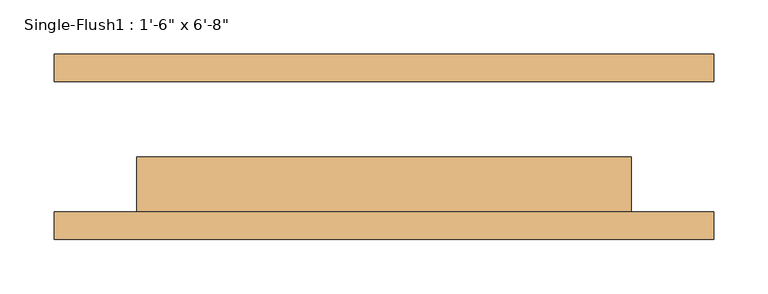
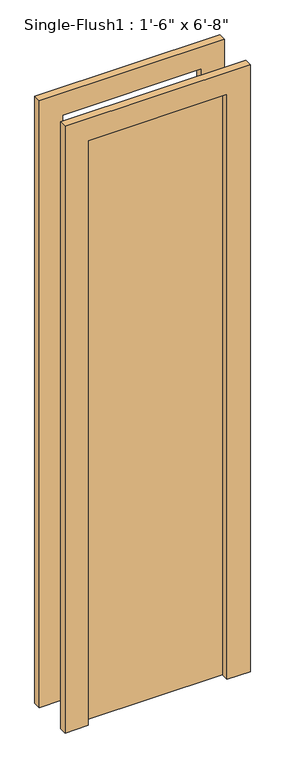
"""IFC4 building model written with IfcOpenShell, lengths in millimetres: door geometry."""

import ifcopenshell
import ifcopenshell.guid

model = None  # the IFC model being written
_history = None  # IfcOwnerHistory: only IFC2X3 demands one
_inside = {}  # id of a spatial element -> (the spatial element, [elements in it])
_under = {}  # id of a project, library or spatial element -> (it, [spatial elements below it])
_declared = {}  # id of a project -> (the project, [libraries it declares])
_typed = {}  # id of a type object -> (the type object, [elements of that type])
_made_of = {}  # id of a material, layer set ... -> (it, [elements and type objects made of it])


def new_model(schema):
    """Start an empty IFC model of exactly this schema.

    Asked for "IFC4X3", IfcOpenShell would pick the latest addendum, in which some entities
    have other attributes; the version numbers below select the first issue.
    IFC2X3 requires an IfcOwnerHistory on every rooted entity: one is made here for all.
    """
    global model, _history
    if schema == "IFC4X3":
        model = ifcopenshell.file(schema_version=(4, 3, 0, 0))
    else:
        model = ifcopenshell.file(schema=schema)
    _inside.clear()
    _under.clear()
    _declared.clear()
    _typed.clear()
    _made_of.clear()
    _history = None
    if model.schema == "IFC2X3":
        org = make("IfcOrganization", Name="unknown")
        user = make(
            "IfcPersonAndOrganization",
            ThePerson=make("IfcPerson", FamilyName="unknown"),
            TheOrganization=org,
        )
        app = make(
            "IfcApplication",
            ApplicationDeveloper=org,
            Version="unknown",
            ApplicationFullName="unknown",
            ApplicationIdentifier="unknown",
        )
        _history = make(
            "IfcOwnerHistory",
            OwningUser=user,
            OwningApplication=app,
            ChangeAction="ADDED",
            CreationDate=0,
        )
    return model


def make(cls, **values):
    """One entity of the class cls with the attributes given. An attribute that is None is left unset."""
    return model.create_entity(
        cls, **{name: value for name, value in values.items() if value is not None}
    )


def rooted(cls, **values):
    """An entity with a GlobalId (a new one), such as an element, a storey or a relation."""
    return make(cls, GlobalId=ifcopenshell.guid.new(), OwnerHistory=_history, **values)


def si_unit(unit_type, name, prefix=None):
    """IfcSIUnit, for example si_unit("LENGTHUNIT", "METRE", prefix="MILLI")."""
    return make("IfcSIUnit", UnitType=unit_type, Prefix=prefix, Name=name)


def assignment(units):
    """IfcUnitAssignment: the units of a project."""
    return None if units is None else make("IfcUnitAssignment", Units=units)


def point(xyz):
    """IfcCartesianPoint."""
    return None if xyz is None else make("IfcCartesianPoint", Coordinates=xyz)


def direction(xyz):
    """IfcDirection."""
    return None if xyz is None else make("IfcDirection", DirectionRatios=xyz)


def frame(location, z_axis=None, x_axis=None):
    """IfcAxis2Placement3D, a coordinate frame: its origin and axes. An axis left out is left unset."""
    return make(
        "IfcAxis2Placement3D",
        Location=point(location),
        Axis=direction(z_axis),
        RefDirection=direction(x_axis),
    )


def origin():
    """The frame at (0, 0, 0) with its axes left unset."""
    return frame((0.0, 0.0, 0.0))


def origin_with_axes():
    """The frame at (0, 0, 0) with the z axis (0, 0, 1) and the x axis (1, 0, 0) written out."""
    return frame((0.0, 0.0, 0.0), z_axis=(0.0, 0.0, 1.0), x_axis=(1.0, 0.0, 0.0))


def place(relative_to, where):
    """IfcLocalPlacement: puts the frame where relative to a parent placement (None: the world)."""
    return make(
        "IfcLocalPlacement", PlacementRelTo=relative_to, RelativePlacement=where
    )


def context(
    kind, dimensions, precision=None, world=None, true_north=None, identifier=None
):
    """IfcGeometricRepresentationContext, for example the 3D "Model" context."""
    return make(
        "IfcGeometricRepresentationContext",
        ContextIdentifier=identifier,
        ContextType=kind,
        CoordinateSpaceDimension=dimensions,
        Precision=precision,
        WorldCoordinateSystem=world,
        TrueNorth=true_north,
    )


def project(units=None, contexts=None):
    """IfcProject with its units and contexts."""
    return rooted(
        "IfcProject",
        Name="project",
        RepresentationContexts=contexts,
        UnitsInContext=assignment(units),
    )


def spatial(cls, under=None, at=None, **own):
    """A site, building, storey or space (cls), placed at a placement, below another one or the project."""
    s = rooted(cls, ObjectPlacement=at, **own)
    if under is not None:
        _under.setdefault(under.id(), (under, []))[1].append(s)
    return s


def polyline(points):
    """IfcPolyline through the points."""
    return make("IfcPolyline", Points=[point(p) for p in points])


def outline(outer, holes=None, kind="AREA"):
    """IfcArbitraryClosedProfileDef: a profile drawn as a closed curve; with holes, ...WithVoids."""
    if holes is None:
        return make("IfcArbitraryClosedProfileDef", ProfileType=kind, OuterCurve=outer)
    return make(
        "IfcArbitraryProfileDefWithVoids",
        ProfileType=kind,
        OuterCurve=outer,
        InnerCurves=holes,
    )


def extrude(swept, where, along, depth):
    """IfcExtrudedAreaSolid: the profile swept, set in the frame where, extruded along a direction by depth."""
    return make(
        "IfcExtrudedAreaSolid",
        SweptArea=swept,
        Position=where,
        ExtrudedDirection=direction(along),
        Depth=depth,
    )


def shape(context_of_items, identifier, shape_type, items):
    """IfcShapeRepresentation: the items that make up one representation, for example the "Body"."""
    return make(
        "IfcShapeRepresentation",
        ContextOfItems=context_of_items,
        RepresentationIdentifier=identifier,
        RepresentationType=shape_type,
        Items=items,
    )


def source(mapping_origin, context_of_items, identifier, shape_type, items):
    """IfcRepresentationMap: a shape defined once, which mapped items show again and again."""
    return make(
        "IfcRepresentationMap",
        MappingOrigin=mapping_origin,
        MappedRepresentation=shape(context_of_items, identifier, shape_type, items),
    )


def transform(
    local_origin,
    x_axis=None,
    y_axis=None,
    z_axis=None,
    scale=None,
    scale2=None,
    scale3=None,
    uniform=True,
):
    """IfcCartesianTransformationOperator3D, or its non-uniform kind. x_axis, y_axis, z_axis: its Axis1, 2, 3."""
    if uniform:
        return make(
            "IfcCartesianTransformationOperator3D",
            Axis1=direction(x_axis),
            Axis2=direction(y_axis),
            LocalOrigin=point(local_origin),
            Scale=scale,
            Axis3=direction(z_axis),
        )
    return make(
        "IfcCartesianTransformationOperator3DnonUniform",
        Axis1=direction(x_axis),
        Axis2=direction(y_axis),
        LocalOrigin=point(local_origin),
        Scale=scale,
        Axis3=direction(z_axis),
        Scale2=scale2,
        Scale3=scale3,
    )


def mapped(mapping_source, mapping_target):
    """IfcMappedItem: shows the shape of a source again, moved by a transform."""
    return make(
        "IfcMappedItem", MappingSource=mapping_source, MappingTarget=mapping_target
    )


def made_of(thing, what):
    """Note that an element or type object is made of a material, layer set ...; save() writes the relation."""
    if what is not None:
        _made_of.setdefault(what.id(), (what, []))[1].append(thing)
    return thing


def element(
    cls,
    number,
    at=None,
    inside=None,
    cuts=None,
    type_object=None,
    material=None,
    context=None,
    identifier="Body",
    shape_type=None,
    held_by="IfcProductDefinitionShape",
    body=None,
    shapes=None,
    **own,
):
    """One element of the class cls, such as IfcWall. Its Tag is "e" and its number.

    at: its placement. inside: the storey or other place that contains it. cuts: it is an
    opening in that element (IfcRelVoidsElement). A single representation is given by context,
    identifier, shape_type and body (its items); several are given by shapes. held_by: the class
    of the entity that holds the representations. save() writes the other relations.
    """
    e = rooted(cls, Tag="e%d" % number, ObjectPlacement=at, **own)
    if body is not None:
        shapes = [shape(context, identifier, shape_type, body)]
    if shapes is not None:
        e.Representation = make(held_by, Representations=shapes)
    if inside is not None:
        _inside.setdefault(inside.id(), (inside, []))[1].append(e)
    if cuts is not None:
        rooted(
            "IfcRelVoidsElement", RelatingBuildingElement=cuts, RelatedOpeningElement=e
        )
    if type_object is not None:
        _typed.setdefault(type_object.id(), (type_object, []))[1].append(e)
    return made_of(e, material)


def aggregate(whole, parts):
    """IfcRelAggregates: a whole, such as a stair, and the parts it consists of."""
    return rooted("IfcRelAggregates", RelatingObject=whole, RelatedObjects=parts)


def save(model, path):
    """Write the relations noted so far, then the file.

    IfcRelAggregates (storeys below a building ...), IfcRelContainedInSpatialStructure (elements
    in a storey), IfcRelDefinesByType, IfcRelAssociatesMaterial and IfcRelDeclares: one each for
    every whole, place, type object, material and project.
    """
    for whole, parts in _under.values():
        aggregate(whole, parts)
    for where, things in _inside.values():
        rooted(
            "IfcRelContainedInSpatialStructure",
            RelatedElements=things,
            RelatingStructure=where,
        )
    for kind, things in _typed.values():
        rooted("IfcRelDefinesByType", RelatedObjects=things, RelatingType=kind)
    for what, things in _made_of.values():
        rooted("IfcRelAssociatesMaterial", RelatedObjects=things, RelatingMaterial=what)
    for by, libraries in _declared.values():
        rooted("IfcRelDeclares", RelatingContext=by, RelatedDefinitions=libraries)
    model.write(path)


def door_8bf1a118(model_context):
    return source(origin(), model_context, "Body", "SweptSolid", [
        extrude(outline(polyline([(2108.2, -304.8), (0.0, -304.8), (0.0, -228.6), (2032.0, -228.6), (2032.0, 228.6), (0.0, 228.6), (0.0, 304.8), (2108.2, 304.8), (2108.2, -304.8)])), frame((0.0, -85.725, 0.0), z_axis=(0.0, 1.0, 0.0), x_axis=(0.0, 0.0, 1.0)), (0.0, 0.0, 1.0), 25.4),
        extrude(outline(polyline([(2108.2, 304.8), (2108.2, -304.8), (0.0, -304.8), (0.0, -228.6), (2032.0, -228.6), (2032.0, 228.6), (0.0, 228.6), (0.0, 304.8), (2108.2, 304.8)])), frame((0.0, 60.325, 0.0), z_axis=(0.0, 1.0, 0.0), x_axis=(0.0, 0.0, 1.0)), (0.0, 0.0, 1.0), 25.4),
        extrude(outline(polyline([(228.6, -9.525), (228.6, -60.325), (-228.6, -60.325), (-228.6, -9.525), (228.6, -9.525)])), origin_with_axes(), (0.0, 0.0, 1.0), 2032.0),
    ])


if __name__ == "__main__":
    model = new_model("IFC4")
    model_context = context("Model", 3, world=origin())
    ifc_project = project(units=[si_unit("LENGTHUNIT", "METRE", prefix="MILLI")], contexts=[model_context])
    site = spatial("IfcSite", under=ifc_project)
    building = spatial("IfcBuilding", under=site)
    placement = place(None, origin())
    door_shape = door_8bf1a118(model_context)
    element("IfcDoor", 1, ObjectType="Single-Flush1 : 1'-6\" x 6'-8\"", at=placement, inside=building, context=model_context, shape_type="MappedRepresentation", body=[
        mapped(door_shape, transform((0.0, 0.0, 0.0), x_axis=(1.0, 0.0, 0.0), y_axis=(0.0, 1.0, 0.0), z_axis=(0.0, 0.0, 1.0))),
    ])
    save(model, "model.ifc")

# Revit data of these elements
# Type "Single-Flush1 : 1'-6\" x 6'-8\""
#   Type Mark = "24"
#   Construction Type Id = "MDOOR"
#   Assembly Code = "C1020"
#   Analytic Construction = "Metal"
#   Thickness = 0' - 2"
#   Heat Transfer Coefficient (U) = 3.7021 W/(m²·K)
#   Height = 6' - 8"
#   Trim Projection Ext = 0' - 1"
#   Trim Projection Int = 0' - 1"
#   Trim Width = 0' - 3"
#   Width = 1' - 6"
#   Door Material = Door - Panel
#   Frame Material = Door - Frame
#   Visual Light Transmittance = 0
#   Solar Heat Gain Coefficient = 0
#   Function = (empty or 0)
#   Wall Closure = (empty or 0)
# Element 1 (IfcDoor, "Single-Flush1 : 1'-6\" x 6'-8\"")
#   Materials on its faces: "Door - Frame", "Door - Panel"
# Materials
#   "Door - Panel": class "Wood", colour RGB 210 159 95, transparency 0, Cost = 0
#   "Door - Frame": class "Miscellaneous", colour RGB 118 70 51, transparency 0, Cost = 0
